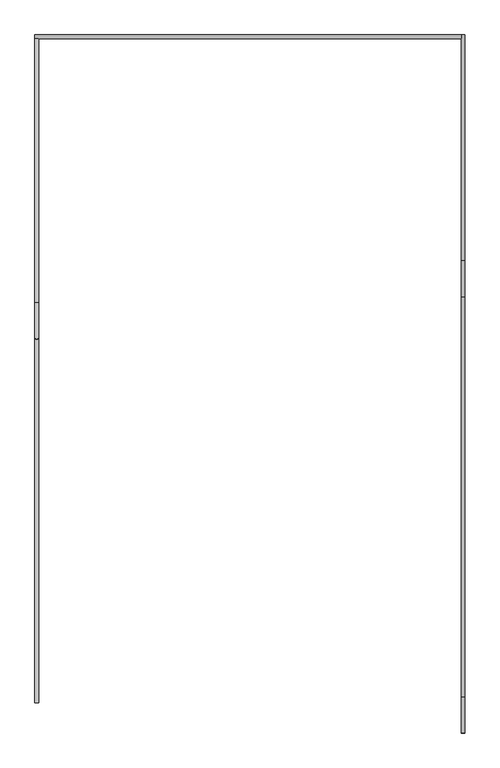
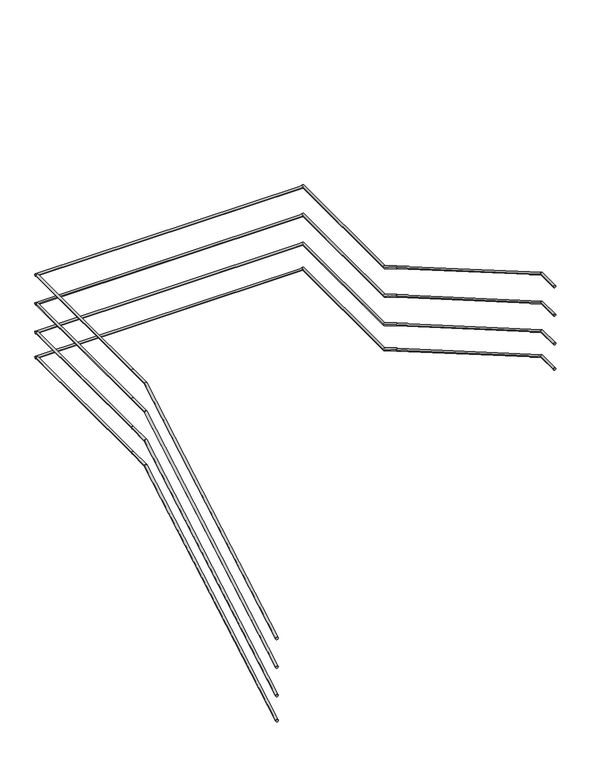
"""IFC4 building model written with IfcOpenShell, lengths in millimetres: railing geometry."""

import ifcopenshell
import ifcopenshell.guid

model = None  # the IFC model being written
_history = None  # IfcOwnerHistory: only IFC2X3 demands one
_inside = {}  # id of a spatial element -> (the spatial element, [elements in it])
_under = {}  # id of a project, library or spatial element -> (it, [spatial elements below it])
_declared = {}  # id of a project -> (the project, [libraries it declares])
_typed = {}  # id of a type object -> (the type object, [elements of that type])
_made_of = {}  # id of a material, layer set ... -> (it, [elements and type objects made of it])


def new_model(schema):
    """Start an empty IFC model of exactly this schema.

    Asked for "IFC4X3", IfcOpenShell would pick the latest addendum, in which some entities
    have other attributes; the version numbers below select the first issue.
    IFC2X3 requires an IfcOwnerHistory on every rooted entity: one is made here for all.
    """
    global model, _history
    if schema == "IFC4X3":
        model = ifcopenshell.file(schema_version=(4, 3, 0, 0))
    else:
        model = ifcopenshell.file(schema=schema)
    _inside.clear()
    _under.clear()
    _declared.clear()
    _typed.clear()
    _made_of.clear()
    _history = None
    if model.schema == "IFC2X3":
        org = make("IfcOrganization", Name="unknown")
        user = make(
            "IfcPersonAndOrganization",
            ThePerson=make("IfcPerson", FamilyName="unknown"),
            TheOrganization=org,
        )
        app = make(
            "IfcApplication",
            ApplicationDeveloper=org,
            Version="unknown",
            ApplicationFullName="unknown",
            ApplicationIdentifier="unknown",
        )
        _history = make(
            "IfcOwnerHistory",
            OwningUser=user,
            OwningApplication=app,
            ChangeAction="ADDED",
            CreationDate=0,
        )
    return model


def make(cls, **values):
    """One entity of the class cls with the attributes given. An attribute that is None is left unset."""
    return model.create_entity(
        cls, **{name: value for name, value in values.items() if value is not None}
    )


def rooted(cls, **values):
    """An entity with a GlobalId (a new one), such as an element, a storey or a relation."""
    return make(cls, GlobalId=ifcopenshell.guid.new(), OwnerHistory=_history, **values)


def si_unit(unit_type, name, prefix=None):
    """IfcSIUnit, for example si_unit("LENGTHUNIT", "METRE", prefix="MILLI")."""
    return make("IfcSIUnit", UnitType=unit_type, Prefix=prefix, Name=name)


def assignment(units):
    """IfcUnitAssignment: the units of a project."""
    return None if units is None else make("IfcUnitAssignment", Units=units)


def point(xyz):
    """IfcCartesianPoint."""
    return None if xyz is None else make("IfcCartesianPoint", Coordinates=xyz)


def direction(xyz):
    """IfcDirection."""
    return None if xyz is None else make("IfcDirection", DirectionRatios=xyz)


def frame(location, z_axis=None, x_axis=None):
    """IfcAxis2Placement3D, a coordinate frame: its origin and axes. An axis left out is left unset."""
    return make(
        "IfcAxis2Placement3D",
        Location=point(location),
        Axis=direction(z_axis),
        RefDirection=direction(x_axis),
    )


def origin():
    """The frame at (0, 0, 0) with its axes left unset."""
    return frame((0.0, 0.0, 0.0))


def place(relative_to, where):
    """IfcLocalPlacement: puts the frame where relative to a parent placement (None: the world)."""
    return make(
        "IfcLocalPlacement", PlacementRelTo=relative_to, RelativePlacement=where
    )


def context(
    kind, dimensions, precision=None, world=None, true_north=None, identifier=None
):
    """IfcGeometricRepresentationContext, for example the 3D "Model" context."""
    return make(
        "IfcGeometricRepresentationContext",
        ContextIdentifier=identifier,
        ContextType=kind,
        CoordinateSpaceDimension=dimensions,
        Precision=precision,
        WorldCoordinateSystem=world,
        TrueNorth=true_north,
    )


def project(units=None, contexts=None):
    """IfcProject with its units and contexts."""
    return rooted(
        "IfcProject",
        Name="project",
        RepresentationContexts=contexts,
        UnitsInContext=assignment(units),
    )


def spatial(cls, under=None, at=None, **own):
    """A site, building, storey or space (cls), placed at a placement, below another one or the project."""
    s = rooted(cls, ObjectPlacement=at, **own)
    if under is not None:
        _under.setdefault(under.id(), (under, []))[1].append(s)
    return s


def circle_curve(where, radius):
    """IfcCircle in the frame where."""
    return make("IfcCircle", Position=where, Radius=radius)


def ellipse_curve(where, semi_axis1, semi_axis2):
    """IfcEllipse in the frame where."""
    return make(
        "IfcEllipse", Position=where, SemiAxis1=semi_axis1, SemiAxis2=semi_axis2
    )


def shape(context_of_items, identifier, shape_type, items):
    """IfcShapeRepresentation: the items that make up one representation, for example the "Body"."""
    return make(
        "IfcShapeRepresentation",
        ContextOfItems=context_of_items,
        RepresentationIdentifier=identifier,
        RepresentationType=shape_type,
        Items=items,
    )


def source(mapping_origin, context_of_items, identifier, shape_type, items):
    """IfcRepresentationMap: a shape defined once, which mapped items show again and again."""
    return make(
        "IfcRepresentationMap",
        MappingOrigin=mapping_origin,
        MappedRepresentation=shape(context_of_items, identifier, shape_type, items),
    )


def transform(
    local_origin,
    x_axis=None,
    y_axis=None,
    z_axis=None,
    scale=None,
    scale2=None,
    scale3=None,
    uniform=True,
):
    """IfcCartesianTransformationOperator3D, or its non-uniform kind. x_axis, y_axis, z_axis: its Axis1, 2, 3."""
    if uniform:
        return make(
            "IfcCartesianTransformationOperator3D",
            Axis1=direction(x_axis),
            Axis2=direction(y_axis),
            LocalOrigin=point(local_origin),
            Scale=scale,
            Axis3=direction(z_axis),
        )
    return make(
        "IfcCartesianTransformationOperator3DnonUniform",
        Axis1=direction(x_axis),
        Axis2=direction(y_axis),
        LocalOrigin=point(local_origin),
        Scale=scale,
        Axis3=direction(z_axis),
        Scale2=scale2,
        Scale3=scale3,
    )


def mapped(mapping_source, mapping_target):
    """IfcMappedItem: shows the shape of a source again, moved by a transform."""
    return make(
        "IfcMappedItem", MappingSource=mapping_source, MappingTarget=mapping_target
    )


def made_of(thing, what):
    """Note that an element or type object is made of a material, layer set ...; save() writes the relation."""
    if what is not None:
        _made_of.setdefault(what.id(), (what, []))[1].append(thing)
    return thing


def element(
    cls,
    number,
    at=None,
    inside=None,
    cuts=None,
    type_object=None,
    material=None,
    context=None,
    identifier="Body",
    shape_type=None,
    held_by="IfcProductDefinitionShape",
    body=None,
    shapes=None,
    **own,
):
    """One element of the class cls, such as IfcWall. Its Tag is "e" and its number.

    at: its placement. inside: the storey or other place that contains it. cuts: it is an
    opening in that element (IfcRelVoidsElement). A single representation is given by context,
    identifier, shape_type and body (its items); several are given by shapes. held_by: the class
    of the entity that holds the representations. save() writes the other relations.
    """
    e = rooted(cls, Tag="e%d" % number, ObjectPlacement=at, **own)
    if body is not None:
        shapes = [shape(context, identifier, shape_type, body)]
    if shapes is not None:
        e.Representation = make(held_by, Representations=shapes)
    if inside is not None:
        _inside.setdefault(inside.id(), (inside, []))[1].append(e)
    if cuts is not None:
        rooted(
            "IfcRelVoidsElement", RelatingBuildingElement=cuts, RelatedOpeningElement=e
        )
    if type_object is not None:
        _typed.setdefault(type_object.id(), (type_object, []))[1].append(e)
    return made_of(e, material)


def aggregate(whole, parts):
    """IfcRelAggregates: a whole, such as a stair, and the parts it consists of."""
    return rooted("IfcRelAggregates", RelatingObject=whole, RelatedObjects=parts)


def save(model, path):
    """Write the relations noted so far, then the file.

    IfcRelAggregates (storeys below a building ...), IfcRelContainedInSpatialStructure (elements
    in a storey), IfcRelDefinesByType, IfcRelAssociatesMaterial and IfcRelDeclares: one each for
    every whole, place, type object, material and project.
    """
    for whole, parts in _under.values():
        aggregate(whole, parts)
    for where, things in _inside.values():
        rooted(
            "IfcRelContainedInSpatialStructure",
            RelatedElements=things,
            RelatingStructure=where,
        )
    for kind, things in _typed.values():
        rooted("IfcRelDefinesByType", RelatedObjects=things, RelatingType=kind)
    for what, things in _made_of.values():
        rooted("IfcRelAssociatesMaterial", RelatedObjects=things, RelatingMaterial=what)
    for by, libraries in _declared.values():
        rooted("IfcRelDeclares", RelatingContext=by, RelatedDefinitions=libraries)
    model.write(path)


def plane_surface(at):
    """IfcPlane: the flat surface through the origin of the frame at, square to its z axis."""
    return make("IfcPlane", Position=at)


def cylinder_surface(at, radius):
    """IfcCylindricalSurface: all points at the distance radius from the z axis of the frame at."""
    return make("IfcCylindricalSurface", Position=at, Radius=radius)


def advanced_brep(points, edges, surfaces, faces):
    """IfcAdvancedBrep: a solid bounded by faces that lie on surfaces and meet in shared edges.

    An edge is (start, end): straight between two places in points (the first is 0);
    or (start, end, curve); or (start, end, curve, False) where it runs against its curve.
    A face is (place in surfaces, loops), or (place, loops, False) where it looks against
    its surface's normal. A loop lists edges by number (the first is 1), with a minus sign
    where the edge is run from its end to its start. The first loop is the outer one.
    """
    corners = [point(p) for p in points]
    vertices = [make("IfcVertexPoint", VertexGeometry=c) for c in corners]
    made = []
    for start, end, *more in edges:
        made.append(
            make(
                "IfcEdgeCurve",
                EdgeStart=vertices[start],
                EdgeEnd=vertices[end],
                EdgeGeometry=more[0] if more else make("IfcPolyline", Points=[corners[start], corners[end]]),
                SameSense=more[1] if len(more) > 1 else True,
            )
        )
    hull = []
    for where, loops, *sense in faces:
        bounds = []
        for j, loop in enumerate(loops):
            ring = [make("IfcOrientedEdge", EdgeElement=made[abs(k) - 1], Orientation=k > 0) for k in loop]
            bounds.append(
                make(
                    "IfcFaceOuterBound" if j == 0 else "IfcFaceBound",
                    Bound=make("IfcEdgeLoop", EdgeList=ring),
                    Orientation=True,
                )
            )
        hull.append(make("IfcAdvancedFace", Bounds=bounds, FaceSurface=surfaces[where], SameSense=sense[0] if sense else True))
    return make("IfcAdvancedBrep", Outer=make("IfcClosedShell", CfsFaces=hull))


def railing_27d6a30b(model_context):
    return source(origin(), model_context, "Body", "AdvancedBrep", [
        advanced_brep(
        [(51115.4, 12029.5208589, 12766.5366726), (51085.4, 12029.5208589, 12766.5366726), (51115.4, 15033.554313, 14508.0053416), (51085.4, 15033.554313, 14508.0053416), (51115.4, 15329.5208589, 14508.0053416), (51085.4, 15329.5208589, 14508.0053416)],
        [
            (0, 1, ellipse_curve(frame((51100.4, 12029.5208589, 12766.5366726), z_axis=(0.0, -1.0, 0.0), x_axis=(0.0, 0.0, -1.0)), 17.3382342, 15.0)),
            (1, 0, ellipse_curve(frame((51100.4, 12029.5208589, 12766.5366726), z_axis=(0.0, -1.0, 0.0), x_axis=(0.0, 0.0, -1.0)), 17.3382342, 15.0)),
            (0, 2),
            (2, 3, ellipse_curve(frame((51100.4, 15033.554313, 14508.0053416), z_axis=(0.0, -0.9656966401166088, -0.25967286971782944), x_axis=(0.0, 0.25967286971782905, -0.9656966401166089)), 15.5328282, 15.0)),
            (3, 1),
            (3, 2, ellipse_curve(frame((51100.4, 15033.554313, 14508.0053416), z_axis=(0.0, -0.9656966401166088, -0.25967286971782944), x_axis=(0.0, 0.25967286971782905, -0.9656966401166089)), 15.5328282, 15.0)),
            (4, 5, circle_curve(frame((51100.4, 15329.5208589, 14508.0053416), z_axis=(0.0, 1.0, 0.0), x_axis=(-1.0, 0.0, 0.0)), 15.0)),
            (5, 4, circle_curve(frame((51100.4, 15329.5208589, 14508.0053416), z_axis=(0.0, 1.0, 0.0), x_axis=(-1.0, 0.0, 0.0)), 15.0)),
            (2, 4),
            (5, 3),
        ],
        [
            plane_surface(frame((51100.4, 12029.5208589, 12783.8749068), z_axis=(0.0, -1.0, 0.0), x_axis=(0.0, 0.0, 1.0))),
            cylinder_surface(frame((51100.4, 12037.0438154, 12770.8978068), z_axis=(0.0, -0.8651400014650144, -0.5015304356318916), x_axis=(-1.0, 0.0, 0.0)), 15.0),
            plane_surface(frame((51100.4, 15329.5208589, 14523.0053416), z_axis=(0.0, 1.0, 0.0), x_axis=(0.0, 0.0, 1.0))),
            cylinder_surface(frame((51100.4, 15029.5208589, 14508.0053416), z_axis=(0.0, -1.0, 0.0), x_axis=(-1.0, 0.0, 0.0)), 15.0),
        ],
        [
            (0, [[1, 2]]),
            (1, [[-1, 3, 4, 5]]),
            (1, [[-2, -5, 6, -3]]),
            (2, [[7, 8]]),
            (3, [[-4, 9, -8, 10]]),
            (3, [[-6, -10, -7, -9]]),
        ],
    ),
        advanced_brep(
        [(51115.4, 15329.5208589, 14508.0053416), (51085.4, 15329.5208589, 14508.0053416), (51115.4, 17509.1208589, 14508.0053416), (51085.4, 17509.1208589, 14508.0053416)],
        [
            (0, 1, circle_curve(frame((51100.4, 15329.5208589, 14508.0053416), z_axis=(0.0, -1.0, 0.0), x_axis=(-1.0, 0.0, 0.0)), 15.0)),
            (1, 0, circle_curve(frame((51100.4, 15329.5208589, 14508.0053416), z_axis=(0.0, -1.0, 0.0), x_axis=(-1.0, 0.0, 0.0)), 15.0)),
            (2, 3, circle_curve(frame((51100.4, 17509.1208589, 14508.0053416), z_axis=(0.0, 1.0, 0.0), x_axis=(-1.0, 0.0, 0.0)), 15.0)),
            (3, 2, circle_curve(frame((51100.4, 17509.1208589, 14508.0053416), z_axis=(0.0, 1.0, 0.0), x_axis=(-1.0, 0.0, 0.0)), 15.0)),
            (0, 2),
            (3, 1),
        ],
        [
            plane_surface(frame((51100.4, 15329.5208589, 14523.0053416), z_axis=(0.0, -1.0, 0.0), x_axis=(0.0, 0.0, 1.0))),
            plane_surface(frame((51100.4, 17509.1208589, 14523.0053416), z_axis=(0.0, 1.0, 0.0), x_axis=(0.0, 0.0, 1.0))),
            cylinder_surface(frame((51100.4, 15329.5208589, 14508.0053416), z_axis=(0.0, -1.0, 0.0), x_axis=(-1.0, 0.0, 0.0)), 15.0),
        ],
        [
            (0, [[1, 2]]),
            (1, [[3, 4]]),
            (2, [[-1, 5, -4, 6]]),
            (2, [[-2, -6, -3, -5]]),
        ],
    ),
        advanced_brep(
        [(51085.4, 17509.1208589, 14508.0053416), (51085.4, 17539.1208589, 14508.0053416), (54606.835546, 17509.1208589, 14508.0053416), (54606.835546, 17539.1208589, 14508.0053416)],
        [
            (0, 1, circle_curve(frame((51085.4, 17524.1208589, 14508.0053416), z_axis=(-1.0, 0.0, 0.0), x_axis=(0.0, 1.0, 0.0)), 15.0)),
            (1, 0, circle_curve(frame((51085.4, 17524.1208589, 14508.0053416), z_axis=(-1.0, 0.0, 0.0), x_axis=(0.0, 1.0, 0.0)), 15.0)),
            (2, 3, circle_curve(frame((54606.835546, 17524.1208589, 14508.0053416), z_axis=(1.0, 0.0, 0.0), x_axis=(0.0, 1.0, 0.0)), 15.0)),
            (3, 2, circle_curve(frame((54606.835546, 17524.1208589, 14508.0053416), z_axis=(1.0, 0.0, 0.0), x_axis=(0.0, 1.0, 0.0)), 15.0)),
            (0, 2),
            (3, 1),
        ],
        [
            plane_surface(frame((51085.4, 17524.1208589, 14523.0053416), z_axis=(-1.0, 0.0, 0.0), x_axis=(0.0, 1.0, 0.0))),
            plane_surface(frame((54606.835546, 17524.1208589, 14523.0053416), z_axis=(1.0, 0.0, 0.0), x_axis=(0.0, 1.0, 0.0))),
            cylinder_surface(frame((51085.4, 17524.1208589, 14508.0053416), z_axis=(-1.0, 0.0, 0.0), x_axis=(0.0, 1.0, 0.0)), 15.0),
        ],
        [
            (0, [[1, 2]]),
            (1, [[3, 4]]),
            (2, [[-1, 5, -4, 6]]),
            (2, [[-2, -6, -3, -5]]),
        ],
    ),
        advanced_brep(
        [(54606.835546, 17539.1208589, 14508.0053416), (54636.835546, 17539.1208589, 14508.0053416), (54606.835546, 15675.4874048, 14508.0053416), (54636.835546, 15675.4874048, 14508.0053416), (54606.835546, 15379.5208589, 14679.5801509), (54636.835546, 15379.5208589, 14679.5801509)],
        [
            (0, 1, circle_curve(frame((54621.835546, 17539.1208589, 14508.0053416), z_axis=(0.0, 1.0, 0.0), x_axis=(1.0, 0.0, 0.0)), 15.0)),
            (1, 0, circle_curve(frame((54621.835546, 17539.1208589, 14508.0053416), z_axis=(0.0, 1.0, 0.0), x_axis=(1.0, 0.0, 0.0)), 15.0)),
            (0, 2),
            (2, 3, ellipse_curve(frame((54621.835546, 15675.4874048, 14508.0053416), z_axis=(0.0, 0.9656966401166088, -0.25967286971782944), x_axis=(0.0, 0.2596728697178298, 0.9656966401166087)), 15.5328282, 15.0)),
            (3, 1),
            (3, 2, ellipse_curve(frame((54621.835546, 15675.4874048, 14508.0053416), z_axis=(0.0, 0.9656966401166088, -0.25967286971782944), x_axis=(0.0, 0.2596728697178298, 0.9656966401166087)), 15.5328282, 15.0)),
            (4, 5, ellipse_curve(frame((54621.835546, 15379.5208589, 14679.5801509), z_axis=(0.0, -1.0, 0.0), x_axis=(0.0, 0.0, -1.0)), 17.3382342, 15.0)),
            (5, 4, ellipse_curve(frame((54621.835546, 15379.5208589, 14679.5801509), z_axis=(0.0, -1.0, 0.0), x_axis=(0.0, 0.0, -1.0)), 17.3382342, 15.0)),
            (2, 4),
            (5, 3),
        ],
        [
            plane_surface(frame((54621.835546, 17539.1208589, 14523.0053416), z_axis=(0.0, 1.0, 0.0), x_axis=(0.0, 0.0, -1.0))),
            cylinder_surface(frame((54621.835546, 17539.1208589, 14508.0053416), z_axis=(0.0, 1.0, 0.0), x_axis=(1.0, 0.0, 0.0)), 15.0),
            plane_surface(frame((54621.835546, 15379.5208589, 14696.9183851), z_axis=(0.0, -1.0, 0.0), x_axis=(0.0, 0.0, -1.0))),
            cylinder_surface(frame((54621.835546, 15671.9979024, 14510.0282416), z_axis=(0.0, 0.8651400014650144, -0.5015304356318916), x_axis=(1.0, 0.0, 0.0)), 15.0),
        ],
        [
            (0, [[1, 2]]),
            (1, [[-1, 3, 4, 5]]),
            (1, [[-2, -5, 6, -3]]),
            (2, [[7, 8]]),
            (3, [[-4, 9, -8, 10]]),
            (3, [[-6, -10, -7, -9]]),
        ],
    ),
        advanced_brep(
        [(54606.835546, 15379.5208589, 14679.5801509), (54636.835546, 15379.5208589, 14679.5801509), (54606.835546, 12075.4874048, 16594.9618634), (54636.835546, 12075.4874048, 16594.9618634), (54606.835546, 11779.5208589, 16594.9618634), (54636.835546, 11779.5208589, 16594.9618634)],
        [
            (0, 1, ellipse_curve(frame((54621.835546, 15379.5208589, 14679.5801509), z_axis=(0.0, 1.0, 0.0), x_axis=(0.0, 0.0, -1.0)), 17.3382342, 15.0)),
            (1, 0, ellipse_curve(frame((54621.835546, 15379.5208589, 14679.5801509), z_axis=(0.0, 1.0, 0.0), x_axis=(0.0, 0.0, -1.0)), 17.3382342, 15.0)),
            (0, 2),
            (2, 3, ellipse_curve(frame((54621.835546, 12075.4874048, 16594.9618634), z_axis=(0.0, 0.9656966401166087, -0.2596728697178297), x_axis=(0.0, -0.259672869717829, -0.9656966401166089)), 15.5328282, 15.0)),
            (3, 1),
            (3, 2, ellipse_curve(frame((54621.835546, 12075.4874048, 16594.9618634), z_axis=(0.0, 0.9656966401166087, -0.2596728697178297), x_axis=(0.0, -0.259672869717829, -0.9656966401166089)), 15.5328282, 15.0)),
            (4, 5, circle_curve(frame((54621.835546, 11779.5208589, 16594.9618634), z_axis=(0.0, -1.0, 0.0), x_axis=(1.0, 0.0, 0.0)), 15.0)),
            (5, 4, circle_curve(frame((54621.835546, 11779.5208589, 16594.9618634), z_axis=(0.0, -1.0, 0.0), x_axis=(1.0, 0.0, 0.0)), 15.0)),
            (2, 4),
            (5, 3),
        ],
        [
            plane_surface(frame((54621.835546, 15379.5208589, 14696.9183851), z_axis=(0.0, 1.0, 0.0), x_axis=(0.0, 0.0, -1.0))),
            cylinder_surface(frame((54621.835546, 15371.9979024, 14683.9412851), z_axis=(0.0, 0.865140001465014, -0.5015304356318923), x_axis=(1.0, 0.0, 0.0)), 15.0),
            plane_surface(frame((54621.835546, 11779.5208589, 16609.9618634), z_axis=(0.0, -1.0, 0.0), x_axis=(0.0, 0.0, -1.0))),
            cylinder_surface(frame((54621.835546, 12079.5208589, 16594.9618634), z_axis=(0.0, 1.0, 0.0), x_axis=(1.0, 0.0, 0.0)), 15.0),
        ],
        [
            (0, [[1, 2]]),
            (1, [[-1, 3, 4, 5]]),
            (1, [[-2, -5, 6, -3]]),
            (2, [[7, 8]]),
            (3, [[-4, 9, -8, 10]]),
            (3, [[-6, -10, -7, -9]]),
        ],
    ),
        advanced_brep(
        [(51115.4, 12029.5208589, 11966.5366726), (51085.4, 12029.5208589, 11966.5366726), (51115.4, 15033.554313, 13708.0053416), (51085.4, 15033.554313, 13708.0053416), (51115.4, 15329.5208589, 13708.0053416), (51085.4, 15329.5208589, 13708.0053416)],
        [
            (0, 1, ellipse_curve(frame((51100.4, 12029.5208589, 11966.5366726), z_axis=(0.0, -1.0, 0.0), x_axis=(0.0, 0.0, -1.0)), 17.3382342, 15.0)),
            (1, 0, ellipse_curve(frame((51100.4, 12029.5208589, 11966.5366726), z_axis=(0.0, -1.0, 0.0), x_axis=(0.0, 0.0, -1.0)), 17.3382342, 15.0)),
            (0, 2),
            (2, 3, ellipse_curve(frame((51100.4, 15033.554313, 13708.0053416), z_axis=(0.0, -0.9656966401166088, -0.25967286971782944), x_axis=(0.0, 0.25967286971782905, -0.9656966401166089)), 15.5328282, 15.0)),
            (3, 1),
            (3, 2, ellipse_curve(frame((51100.4, 15033.554313, 13708.0053416), z_axis=(0.0, -0.9656966401166088, -0.25967286971782944), x_axis=(0.0, 0.25967286971782905, -0.9656966401166089)), 15.5328282, 15.0)),
            (4, 5, circle_curve(frame((51100.4, 15329.5208589, 13708.0053416), z_axis=(0.0, 1.0, 0.0), x_axis=(-1.0, 0.0, 0.0)), 15.0)),
            (5, 4, circle_curve(frame((51100.4, 15329.5208589, 13708.0053416), z_axis=(0.0, 1.0, 0.0), x_axis=(-1.0, 0.0, 0.0)), 15.0)),
            (2, 4),
            (5, 3),
        ],
        [
            plane_surface(frame((51100.4, 12029.5208589, 11983.8749068), z_axis=(0.0, -1.0, 0.0), x_axis=(0.0, 0.0, 1.0))),
            cylinder_surface(frame((51100.4, 12037.0438154, 11970.8978068), z_axis=(0.0, -0.8651400014650144, -0.5015304356318916), x_axis=(-1.0, 0.0, 0.0)), 15.0),
            plane_surface(frame((51100.4, 15329.5208589, 13723.0053416), z_axis=(0.0, 1.0, 0.0), x_axis=(0.0, 0.0, 1.0))),
            cylinder_surface(frame((51100.4, 15029.5208589, 13708.0053416), z_axis=(0.0, -1.0, 0.0), x_axis=(-1.0, 0.0, 0.0)), 15.0),
        ],
        [
            (0, [[1, 2]]),
            (1, [[-1, 3, 4, 5]]),
            (1, [[-2, -5, 6, -3]]),
            (2, [[7, 8]]),
            (3, [[-4, 9, -8, 10]]),
            (3, [[-6, -10, -7, -9]]),
        ],
    ),
        advanced_brep(
        [(51115.4, 15329.5208589, 13708.0053416), (51085.4, 15329.5208589, 13708.0053416), (51115.4, 17509.1208589, 13708.0053416), (51085.4, 17509.1208589, 13708.0053416)],
        [
            (0, 1, circle_curve(frame((51100.4, 15329.5208589, 13708.0053416), z_axis=(0.0, -1.0, 0.0), x_axis=(-1.0, 0.0, 0.0)), 15.0)),
            (1, 0, circle_curve(frame((51100.4, 15329.5208589, 13708.0053416), z_axis=(0.0, -1.0, 0.0), x_axis=(-1.0, 0.0, 0.0)), 15.0)),
            (2, 3, circle_curve(frame((51100.4, 17509.1208589, 13708.0053416), z_axis=(0.0, 1.0, 0.0), x_axis=(-1.0, 0.0, 0.0)), 15.0)),
            (3, 2, circle_curve(frame((51100.4, 17509.1208589, 13708.0053416), z_axis=(0.0, 1.0, 0.0), x_axis=(-1.0, 0.0, 0.0)), 15.0)),
            (0, 2),
            (3, 1),
        ],
        [
            plane_surface(frame((51100.4, 15329.5208589, 13723.0053416), z_axis=(0.0, -1.0, 0.0), x_axis=(0.0, 0.0, 1.0))),
            plane_surface(frame((51100.4, 17509.1208589, 13723.0053416), z_axis=(0.0, 1.0, 0.0), x_axis=(0.0, 0.0, 1.0))),
            cylinder_surface(frame((51100.4, 15329.5208589, 13708.0053416), z_axis=(0.0, -1.0, 0.0), x_axis=(-1.0, 0.0, 0.0)), 15.0),
        ],
        [
            (0, [[1, 2]]),
            (1, [[3, 4]]),
            (2, [[-1, 5, -4, 6]]),
            (2, [[-2, -6, -3, -5]]),
        ],
    ),
        advanced_brep(
        [(51085.4, 17509.1208589, 13708.0053416), (51085.4, 17539.1208589, 13708.0053416), (54606.835546, 17509.1208589, 13708.0053416), (54606.835546, 17539.1208589, 13708.0053416)],
        [
            (0, 1, circle_curve(frame((51085.4, 17524.1208589, 13708.0053416), z_axis=(-1.0, 0.0, 0.0), x_axis=(0.0, 1.0, 0.0)), 15.0)),
            (1, 0, circle_curve(frame((51085.4, 17524.1208589, 13708.0053416), z_axis=(-1.0, 0.0, 0.0), x_axis=(0.0, 1.0, 0.0)), 15.0)),
            (2, 3, circle_curve(frame((54606.835546, 17524.1208589, 13708.0053416), z_axis=(1.0, 0.0, 0.0), x_axis=(0.0, 1.0, 0.0)), 15.0)),
            (3, 2, circle_curve(frame((54606.835546, 17524.1208589, 13708.0053416), z_axis=(1.0, 0.0, 0.0), x_axis=(0.0, 1.0, 0.0)), 15.0)),
            (0, 2),
            (3, 1),
        ],
        [
            plane_surface(frame((51085.4, 17524.1208589, 13723.0053416), z_axis=(-1.0, 0.0, 0.0), x_axis=(0.0, 1.0, 0.0))),
            plane_surface(frame((54606.835546, 17524.1208589, 13723.0053416), z_axis=(1.0, 0.0, 0.0), x_axis=(0.0, 1.0, 0.0))),
            cylinder_surface(frame((51085.4, 17524.1208589, 13708.0053416), z_axis=(-1.0, 0.0, 0.0), x_axis=(0.0, 1.0, 0.0)), 15.0),
        ],
        [
            (0, [[1, 2]]),
            (1, [[3, 4]]),
            (2, [[-1, 5, -4, 6]]),
            (2, [[-2, -6, -3, -5]]),
        ],
    ),
        advanced_brep(
        [(54606.835546, 17539.1208589, 13708.0053416), (54636.835546, 17539.1208589, 13708.0053416), (54606.835546, 15675.4874048, 13708.0053416), (54636.835546, 15675.4874048, 13708.0053416), (54606.835546, 15379.5208589, 13879.5801509), (54636.835546, 15379.5208589, 13879.5801509)],
        [
            (0, 1, circle_curve(frame((54621.835546, 17539.1208589, 13708.0053416), z_axis=(0.0, 1.0, 0.0), x_axis=(1.0, 0.0, 0.0)), 15.0)),
            (1, 0, circle_curve(frame((54621.835546, 17539.1208589, 13708.0053416), z_axis=(0.0, 1.0, 0.0), x_axis=(1.0, 0.0, 0.0)), 15.0)),
            (0, 2),
            (2, 3, ellipse_curve(frame((54621.835546, 15675.4874048, 13708.0053416), z_axis=(0.0, 0.9656966401166088, -0.25967286971782944), x_axis=(0.0, 0.2596728697178298, 0.9656966401166087)), 15.5328282, 15.0)),
            (3, 1),
            (3, 2, ellipse_curve(frame((54621.835546, 15675.4874048, 13708.0053416), z_axis=(0.0, 0.9656966401166088, -0.25967286971782944), x_axis=(0.0, 0.2596728697178298, 0.9656966401166087)), 15.5328282, 15.0)),
            (4, 5, ellipse_curve(frame((54621.835546, 15379.5208589, 13879.5801509), z_axis=(0.0, -1.0, 0.0), x_axis=(0.0, 0.0, -1.0)), 17.3382342, 15.0)),
            (5, 4, ellipse_curve(frame((54621.835546, 15379.5208589, 13879.5801509), z_axis=(0.0, -1.0, 0.0), x_axis=(0.0, 0.0, -1.0)), 17.3382342, 15.0)),
            (2, 4),
            (5, 3),
        ],
        [
            plane_surface(frame((54621.835546, 17539.1208589, 13723.0053416), z_axis=(0.0, 1.0, 0.0), x_axis=(0.0, 0.0, -1.0))),
            cylinder_surface(frame((54621.835546, 17539.1208589, 13708.0053416), z_axis=(0.0, 1.0, 0.0), x_axis=(1.0, 0.0, 0.0)), 15.0),
            plane_surface(frame((54621.835546, 15379.5208589, 13896.9183851), z_axis=(0.0, -1.0, 0.0), x_axis=(0.0, 0.0, -1.0))),
            cylinder_surface(frame((54621.835546, 15671.9979024, 13710.0282416), z_axis=(0.0, 0.8651400014650144, -0.5015304356318916), x_axis=(1.0, 0.0, 0.0)), 15.0),
        ],
        [
            (0, [[1, 2]]),
            (1, [[-1, 3, 4, 5]]),
            (1, [[-2, -5, 6, -3]]),
            (2, [[7, 8]]),
            (3, [[-4, 9, -8, 10]]),
            (3, [[-6, -10, -7, -9]]),
        ],
    ),
        advanced_brep(
        [(54606.835546, 15379.5208589, 13879.5801509), (54636.835546, 15379.5208589, 13879.5801509), (54606.835546, 12075.4874048, 15794.9618634), (54636.835546, 12075.4874048, 15794.9618634), (54606.835546, 11779.5208589, 15794.9618634), (54636.835546, 11779.5208589, 15794.9618634)],
        [
            (0, 1, ellipse_curve(frame((54621.835546, 15379.5208589, 13879.5801509), z_axis=(0.0, 1.0, 0.0), x_axis=(0.0, 0.0, -1.0)), 17.3382342, 15.0)),
            (1, 0, ellipse_curve(frame((54621.835546, 15379.5208589, 13879.5801509), z_axis=(0.0, 1.0, 0.0), x_axis=(0.0, 0.0, -1.0)), 17.3382342, 15.0)),
            (0, 2),
            (2, 3, ellipse_curve(frame((54621.835546, 12075.4874048, 15794.9618634), z_axis=(0.0, 0.9656966401166087, -0.2596728697178297), x_axis=(0.0, -0.259672869717829, -0.9656966401166089)), 15.5328282, 15.0)),
            (3, 1),
            (3, 2, ellipse_curve(frame((54621.835546, 12075.4874048, 15794.9618634), z_axis=(0.0, 0.9656966401166087, -0.2596728697178297), x_axis=(0.0, -0.259672869717829, -0.9656966401166089)), 15.5328282, 15.0)),
            (4, 5, circle_curve(frame((54621.835546, 11779.5208589, 15794.9618634), z_axis=(0.0, -1.0, 0.0), x_axis=(1.0, 0.0, 0.0)), 15.0)),
            (5, 4, circle_curve(frame((54621.835546, 11779.5208589, 15794.9618634), z_axis=(0.0, -1.0, 0.0), x_axis=(1.0, 0.0, 0.0)), 15.0)),
            (2, 4),
            (5, 3),
        ],
        [
            plane_surface(frame((54621.835546, 15379.5208589, 13896.9183851), z_axis=(0.0, 1.0, 0.0), x_axis=(0.0, 0.0, -1.0))),
            cylinder_surface(frame((54621.835546, 15371.9979024, 13883.9412851), z_axis=(0.0, 0.865140001465014, -0.5015304356318923), x_axis=(1.0, 0.0, 0.0)), 15.0),
            plane_surface(frame((54621.835546, 11779.5208589, 15809.9618634), z_axis=(0.0, -1.0, 0.0), x_axis=(0.0, 0.0, -1.0))),
            cylinder_surface(frame((54621.835546, 12079.5208589, 15794.9618634), z_axis=(0.0, 1.0, 0.0), x_axis=(1.0, 0.0, 0.0)), 15.0),
        ],
        [
            (0, [[1, 2]]),
            (1, [[-1, 3, 4, 5]]),
            (1, [[-2, -5, 6, -3]]),
            (2, [[7, 8]]),
            (3, [[-4, 9, -8, 10]]),
            (3, [[-6, -10, -7, -9]]),
        ],
    ),
        advanced_brep(
        [(51115.4, 12029.5208589, 12366.5366726), (51085.4, 12029.5208589, 12366.5366726), (51115.4, 15033.554313, 14108.0053416), (51085.4, 15033.554313, 14108.0053416), (51115.4, 15329.5208589, 14108.0053416), (51085.4, 15329.5208589, 14108.0053416)],
        [
            (0, 1, ellipse_curve(frame((51100.4, 12029.5208589, 12366.5366726), z_axis=(0.0, -1.0, 0.0), x_axis=(0.0, 0.0, -1.0)), 17.3382342, 15.0)),
            (1, 0, ellipse_curve(frame((51100.4, 12029.5208589, 12366.5366726), z_axis=(0.0, -1.0, 0.0), x_axis=(0.0, 0.0, -1.0)), 17.3382342, 15.0)),
            (0, 2),
            (2, 3, ellipse_curve(frame((51100.4, 15033.554313, 14108.0053416), z_axis=(0.0, -0.9656966401166088, -0.25967286971782944), x_axis=(0.0, 0.25967286971782905, -0.9656966401166089)), 15.5328282, 15.0)),
            (3, 1),
            (3, 2, ellipse_curve(frame((51100.4, 15033.554313, 14108.0053416), z_axis=(0.0, -0.9656966401166088, -0.25967286971782944), x_axis=(0.0, 0.25967286971782905, -0.9656966401166089)), 15.5328282, 15.0)),
            (4, 5, circle_curve(frame((51100.4, 15329.5208589, 14108.0053416), z_axis=(0.0, 1.0, 0.0), x_axis=(-1.0, 0.0, 0.0)), 15.0)),
            (5, 4, circle_curve(frame((51100.4, 15329.5208589, 14108.0053416), z_axis=(0.0, 1.0, 0.0), x_axis=(-1.0, 0.0, 0.0)), 15.0)),
            (2, 4),
            (5, 3),
        ],
        [
            plane_surface(frame((51100.4, 12029.5208589, 12383.8749068), z_axis=(0.0, -1.0, 0.0), x_axis=(0.0, 0.0, 1.0))),
            cylinder_surface(frame((51100.4, 12037.0438154, 12370.8978068), z_axis=(0.0, -0.8651400014650144, -0.5015304356318916), x_axis=(-1.0, 0.0, 0.0)), 15.0),
            plane_surface(frame((51100.4, 15329.5208589, 14123.0053416), z_axis=(0.0, 1.0, 0.0), x_axis=(0.0, 0.0, 1.0))),
            cylinder_surface(frame((51100.4, 15029.5208589, 14108.0053416), z_axis=(0.0, -1.0, 0.0), x_axis=(-1.0, 0.0, 0.0)), 15.0),
        ],
        [
            (0, [[1, 2]]),
            (1, [[-1, 3, 4, 5]]),
            (1, [[-2, -5, 6, -3]]),
            (2, [[7, 8]]),
            (3, [[-4, 9, -8, 10]]),
            (3, [[-6, -10, -7, -9]]),
        ],
    ),
        advanced_brep(
        [(51115.4, 15329.5208589, 14108.0053416), (51085.4, 15329.5208589, 14108.0053416), (51115.4, 17509.1208589, 14108.0053416), (51085.4, 17509.1208589, 14108.0053416)],
        [
            (0, 1, circle_curve(frame((51100.4, 15329.5208589, 14108.0053416), z_axis=(0.0, -1.0, 0.0), x_axis=(-1.0, 0.0, 0.0)), 15.0)),
            (1, 0, circle_curve(frame((51100.4, 15329.5208589, 14108.0053416), z_axis=(0.0, -1.0, 0.0), x_axis=(-1.0, 0.0, 0.0)), 15.0)),
            (2, 3, circle_curve(frame((51100.4, 17509.1208589, 14108.0053416), z_axis=(0.0, 1.0, 0.0), x_axis=(-1.0, 0.0, 0.0)), 15.0)),
            (3, 2, circle_curve(frame((51100.4, 17509.1208589, 14108.0053416), z_axis=(0.0, 1.0, 0.0), x_axis=(-1.0, 0.0, 0.0)), 15.0)),
            (0, 2),
            (3, 1),
        ],
        [
            plane_surface(frame((51100.4, 15329.5208589, 14123.0053416), z_axis=(0.0, -1.0, 0.0), x_axis=(0.0, 0.0, 1.0))),
            plane_surface(frame((51100.4, 17509.1208589, 14123.0053416), z_axis=(0.0, 1.0, 0.0), x_axis=(0.0, 0.0, 1.0))),
            cylinder_surface(frame((51100.4, 15329.5208589, 14108.0053416), z_axis=(0.0, -1.0, 0.0), x_axis=(-1.0, 0.0, 0.0)), 15.0),
        ],
        [
            (0, [[1, 2]]),
            (1, [[3, 4]]),
            (2, [[-1, 5, -4, 6]]),
            (2, [[-2, -6, -3, -5]]),
        ],
    ),
        advanced_brep(
        [(51085.4, 17509.1208589, 14108.0053416), (51085.4, 17539.1208589, 14108.0053416), (54606.835546, 17509.1208589, 14108.0053416), (54606.835546, 17539.1208589, 14108.0053416)],
        [
            (0, 1, circle_curve(frame((51085.4, 17524.1208589, 14108.0053416), z_axis=(-1.0, 0.0, 0.0), x_axis=(0.0, 1.0, 0.0)), 15.0)),
            (1, 0, circle_curve(frame((51085.4, 17524.1208589, 14108.0053416), z_axis=(-1.0, 0.0, 0.0), x_axis=(0.0, 1.0, 0.0)), 15.0)),
            (2, 3, circle_curve(frame((54606.835546, 17524.1208589, 14108.0053416), z_axis=(1.0, 0.0, 0.0), x_axis=(0.0, 1.0, 0.0)), 15.0)),
            (3, 2, circle_curve(frame((54606.835546, 17524.1208589, 14108.0053416), z_axis=(1.0, 0.0, 0.0), x_axis=(0.0, 1.0, 0.0)), 15.0)),
            (0, 2),
            (3, 1),
        ],
        [
            plane_surface(frame((51085.4, 17524.1208589, 14123.0053416), z_axis=(-1.0, 0.0, 0.0), x_axis=(0.0, 1.0, 0.0))),
            plane_surface(frame((54606.835546, 17524.1208589, 14123.0053416), z_axis=(1.0, 0.0, 0.0), x_axis=(0.0, 1.0, 0.0))),
            cylinder_surface(frame((51085.4, 17524.1208589, 14108.0053416), z_axis=(-1.0, 0.0, 0.0), x_axis=(0.0, 1.0, 0.0)), 15.0),
        ],
        [
            (0, [[1, 2]]),
            (1, [[3, 4]]),
            (2, [[-1, 5, -4, 6]]),
            (2, [[-2, -6, -3, -5]]),
        ],
    ),
        advanced_brep(
        [(54606.835546, 17539.1208589, 14108.0053416), (54636.835546, 17539.1208589, 14108.0053416), (54606.835546, 15675.4874048, 14108.0053416), (54636.835546, 15675.4874048, 14108.0053416), (54606.835546, 15379.5208589, 14279.5801509), (54636.835546, 15379.5208589, 14279.5801509)],
        [
            (0, 1, circle_curve(frame((54621.835546, 17539.1208589, 14108.0053416), z_axis=(0.0, 1.0, 0.0), x_axis=(1.0, 0.0, 0.0)), 15.0)),
            (1, 0, circle_curve(frame((54621.835546, 17539.1208589, 14108.0053416), z_axis=(0.0, 1.0, 0.0), x_axis=(1.0, 0.0, 0.0)), 15.0)),
            (0, 2),
            (2, 3, ellipse_curve(frame((54621.835546, 15675.4874048, 14108.0053416), z_axis=(0.0, 0.9656966401166088, -0.25967286971782944), x_axis=(0.0, 0.2596728697178298, 0.9656966401166087)), 15.5328282, 15.0)),
            (3, 1),
            (3, 2, ellipse_curve(frame((54621.835546, 15675.4874048, 14108.0053416), z_axis=(0.0, 0.9656966401166088, -0.25967286971782944), x_axis=(0.0, 0.2596728697178298, 0.9656966401166087)), 15.5328282, 15.0)),
            (4, 5, ellipse_curve(frame((54621.835546, 15379.5208589, 14279.5801509), z_axis=(0.0, -1.0, 0.0), x_axis=(0.0, 0.0, -1.0)), 17.3382342, 15.0)),
            (5, 4, ellipse_curve(frame((54621.835546, 15379.5208589, 14279.5801509), z_axis=(0.0, -1.0, 0.0), x_axis=(0.0, 0.0, -1.0)), 17.3382342, 15.0)),
            (2, 4),
            (5, 3),
        ],
        [
            plane_surface(frame((54621.835546, 17539.1208589, 14123.0053416), z_axis=(0.0, 1.0, 0.0), x_axis=(0.0, 0.0, -1.0))),
            cylinder_surface(frame((54621.835546, 17539.1208589, 14108.0053416), z_axis=(0.0, 1.0, 0.0), x_axis=(1.0, 0.0, 0.0)), 15.0),
            plane_surface(frame((54621.835546, 15379.5208589, 14296.9183851), z_axis=(0.0, -1.0, 0.0), x_axis=(0.0, 0.0, -1.0))),
            cylinder_surface(frame((54621.835546, 15671.9979024, 14110.0282416), z_axis=(0.0, 0.8651400014650144, -0.5015304356318916), x_axis=(1.0, 0.0, 0.0)), 15.0),
        ],
        [
            (0, [[1, 2]]),
            (1, [[-1, 3, 4, 5]]),
            (1, [[-2, -5, 6, -3]]),
            (2, [[7, 8]]),
            (3, [[-4, 9, -8, 10]]),
            (3, [[-6, -10, -7, -9]]),
        ],
    ),
        advanced_brep(
        [(54606.835546, 15379.5208589, 14279.5801509), (54636.835546, 15379.5208589, 14279.5801509), (54606.835546, 12075.4874048, 16194.9618634), (54636.835546, 12075.4874048, 16194.9618634), (54606.835546, 11779.5208589, 16194.9618634), (54636.835546, 11779.5208589, 16194.9618634)],
        [
            (0, 1, ellipse_curve(frame((54621.835546, 15379.5208589, 14279.5801509), z_axis=(0.0, 1.0, 0.0), x_axis=(0.0, 0.0, -1.0)), 17.3382342, 15.0)),
            (1, 0, ellipse_curve(frame((54621.835546, 15379.5208589, 14279.5801509), z_axis=(0.0, 1.0, 0.0), x_axis=(0.0, 0.0, -1.0)), 17.3382342, 15.0)),
            (0, 2),
            (2, 3, ellipse_curve(frame((54621.835546, 12075.4874048, 16194.9618634), z_axis=(0.0, 0.9656966401166087, -0.2596728697178297), x_axis=(0.0, -0.259672869717829, -0.9656966401166089)), 15.5328282, 15.0)),
            (3, 1),
            (3, 2, ellipse_curve(frame((54621.835546, 12075.4874048, 16194.9618634), z_axis=(0.0, 0.9656966401166087, -0.2596728697178297), x_axis=(0.0, -0.259672869717829, -0.9656966401166089)), 15.5328282, 15.0)),
            (4, 5, circle_curve(frame((54621.835546, 11779.5208589, 16194.9618634), z_axis=(0.0, -1.0, 0.0), x_axis=(1.0, 0.0, 0.0)), 15.0)),
            (5, 4, circle_curve(frame((54621.835546, 11779.5208589, 16194.9618634), z_axis=(0.0, -1.0, 0.0), x_axis=(1.0, 0.0, 0.0)), 15.0)),
            (2, 4),
            (5, 3),
        ],
        [
            plane_surface(frame((54621.835546, 15379.5208589, 14296.9183851), z_axis=(0.0, 1.0, 0.0), x_axis=(0.0, 0.0, -1.0))),
            cylinder_surface(frame((54621.835546, 15371.9979024, 14283.9412851), z_axis=(0.0, 0.865140001465014, -0.5015304356318923), x_axis=(1.0, 0.0, 0.0)), 15.0),
            plane_surface(frame((54621.835546, 11779.5208589, 16209.9618634), z_axis=(0.0, -1.0, 0.0), x_axis=(0.0, 0.0, -1.0))),
            cylinder_surface(frame((54621.835546, 12079.5208589, 16194.9618634), z_axis=(0.0, 1.0, 0.0), x_axis=(1.0, 0.0, 0.0)), 15.0),
        ],
        [
            (0, [[1, 2]]),
            (1, [[-1, 3, 4, 5]]),
            (1, [[-2, -5, 6, -3]]),
            (2, [[7, 8]]),
            (3, [[-4, 9, -8, 10]]),
            (3, [[-6, -10, -7, -9]]),
        ],
    ),
        advanced_brep(
        [(51115.4, 12029.5208589, 11616.5366726), (51085.4, 12029.5208589, 11616.5366726), (51115.4, 15033.554313, 13358.0053416), (51085.4, 15033.554313, 13358.0053416), (51115.4, 15329.5208589, 13358.0053416), (51085.4, 15329.5208589, 13358.0053416)],
        [
            (0, 1, ellipse_curve(frame((51100.4, 12029.5208589, 11616.5366726), z_axis=(0.0, -1.0, 0.0), x_axis=(0.0, 0.0, -1.0)), 17.3382342, 15.0)),
            (1, 0, ellipse_curve(frame((51100.4, 12029.5208589, 11616.5366726), z_axis=(0.0, -1.0, 0.0), x_axis=(0.0, 0.0, -1.0)), 17.3382342, 15.0)),
            (0, 2),
            (2, 3, ellipse_curve(frame((51100.4, 15033.554313, 13358.0053416), z_axis=(0.0, -0.9656966401166088, -0.25967286971782944), x_axis=(0.0, 0.25967286971782905, -0.9656966401166089)), 15.5328282, 15.0)),
            (3, 1),
            (3, 2, ellipse_curve(frame((51100.4, 15033.554313, 13358.0053416), z_axis=(0.0, -0.9656966401166088, -0.25967286971782944), x_axis=(0.0, 0.25967286971782905, -0.9656966401166089)), 15.5328282, 15.0)),
            (4, 5, circle_curve(frame((51100.4, 15329.5208589, 13358.0053416), z_axis=(0.0, 1.0, 0.0), x_axis=(-1.0, 0.0, 0.0)), 15.0)),
            (5, 4, circle_curve(frame((51100.4, 15329.5208589, 13358.0053416), z_axis=(0.0, 1.0, 0.0), x_axis=(-1.0, 0.0, 0.0)), 15.0)),
            (2, 4),
            (5, 3),
        ],
        [
            plane_surface(frame((51100.4, 12029.5208589, 11633.8749068), z_axis=(0.0, -1.0, 0.0), x_axis=(0.0, 0.0, 1.0))),
            cylinder_surface(frame((51100.4, 12037.0438154, 11620.8978068), z_axis=(0.0, -0.8651400014650144, -0.5015304356318916), x_axis=(-1.0, 0.0, 0.0)), 15.0),
            plane_surface(frame((51100.4, 15329.5208589, 13373.0053416), z_axis=(0.0, 1.0, 0.0), x_axis=(0.0, 0.0, 1.0))),
            cylinder_surface(frame((51100.4, 15029.5208589, 13358.0053416), z_axis=(0.0, -1.0, 0.0), x_axis=(-1.0, 0.0, 0.0)), 15.0),
        ],
        [
            (0, [[1, 2]]),
            (1, [[-1, 3, 4, 5]]),
            (1, [[-2, -5, 6, -3]]),
            (2, [[7, 8]]),
            (3, [[-4, 9, -8, 10]]),
            (3, [[-6, -10, -7, -9]]),
        ],
    ),
        advanced_brep(
        [(51115.4, 15329.5208589, 13358.0053416), (51085.4, 15329.5208589, 13358.0053416), (51115.4, 17509.1208589, 13358.0053416), (51085.4, 17509.1208589, 13358.0053416)],
        [
            (0, 1, circle_curve(frame((51100.4, 15329.5208589, 13358.0053416), z_axis=(0.0, -1.0, 0.0), x_axis=(-1.0, 0.0, 0.0)), 15.0)),
            (1, 0, circle_curve(frame((51100.4, 15329.5208589, 13358.0053416), z_axis=(0.0, -1.0, 0.0), x_axis=(-1.0, 0.0, 0.0)), 15.0)),
            (2, 3, circle_curve(frame((51100.4, 17509.1208589, 13358.0053416), z_axis=(0.0, 1.0, 0.0), x_axis=(-1.0, 0.0, 0.0)), 15.0)),
            (3, 2, circle_curve(frame((51100.4, 17509.1208589, 13358.0053416), z_axis=(0.0, 1.0, 0.0), x_axis=(-1.0, 0.0, 0.0)), 15.0)),
            (0, 2),
            (3, 1),
        ],
        [
            plane_surface(frame((51100.4, 15329.5208589, 13373.0053416), z_axis=(0.0, -1.0, 0.0), x_axis=(0.0, 0.0, 1.0))),
            plane_surface(frame((51100.4, 17509.1208589, 13373.0053416), z_axis=(0.0, 1.0, 0.0), x_axis=(0.0, 0.0, 1.0))),
            cylinder_surface(frame((51100.4, 15329.5208589, 13358.0053416), z_axis=(0.0, -1.0, 0.0), x_axis=(-1.0, 0.0, 0.0)), 15.0),
        ],
        [
            (0, [[1, 2]]),
            (1, [[3, 4]]),
            (2, [[-1, 5, -4, 6]]),
            (2, [[-2, -6, -3, -5]]),
        ],
    ),
        advanced_brep(
        [(51085.4, 17509.1208589, 13358.0053416), (51085.4, 17539.1208589, 13358.0053416), (54606.835546, 17509.1208589, 13358.0053416), (54606.835546, 17539.1208589, 13358.0053416)],
        [
            (0, 1, circle_curve(frame((51085.4, 17524.1208589, 13358.0053416), z_axis=(-1.0, 0.0, 0.0), x_axis=(0.0, 1.0, 0.0)), 15.0)),
            (1, 0, circle_curve(frame((51085.4, 17524.1208589, 13358.0053416), z_axis=(-1.0, 0.0, 0.0), x_axis=(0.0, 1.0, 0.0)), 15.0)),
            (2, 3, circle_curve(frame((54606.835546, 17524.1208589, 13358.0053416), z_axis=(1.0, 0.0, 0.0), x_axis=(0.0, 1.0, 0.0)), 15.0)),
            (3, 2, circle_curve(frame((54606.835546, 17524.1208589, 13358.0053416), z_axis=(1.0, 0.0, 0.0), x_axis=(0.0, 1.0, 0.0)), 15.0)),
            (0, 2),
            (3, 1),
        ],
        [
            plane_surface(frame((51085.4, 17524.1208589, 13373.0053416), z_axis=(-1.0, 0.0, 0.0), x_axis=(0.0, 1.0, 0.0))),
            plane_surface(frame((54606.835546, 17524.1208589, 13373.0053416), z_axis=(1.0, 0.0, 0.0), x_axis=(0.0, 1.0, 0.0))),
            cylinder_surface(frame((51085.4, 17524.1208589, 13358.0053416), z_axis=(-1.0, 0.0, 0.0), x_axis=(0.0, 1.0, 0.0)), 15.0),
        ],
        [
            (0, [[1, 2]]),
            (1, [[3, 4]]),
            (2, [[-1, 5, -4, 6]]),
            (2, [[-2, -6, -3, -5]]),
        ],
    ),
        advanced_brep(
        [(54606.835546, 17539.1208589, 13358.0053416), (54636.835546, 17539.1208589, 13358.0053416), (54606.835546, 15675.4874048, 13358.0053416), (54636.835546, 15675.4874048, 13358.0053416), (54606.835546, 15379.5208589, 13529.5801509), (54636.835546, 15379.5208589, 13529.5801509)],
        [
            (0, 1, circle_curve(frame((54621.835546, 17539.1208589, 13358.0053416), z_axis=(0.0, 1.0, 0.0), x_axis=(1.0, 0.0, 0.0)), 15.0)),
            (1, 0, circle_curve(frame((54621.835546, 17539.1208589, 13358.0053416), z_axis=(0.0, 1.0, 0.0), x_axis=(1.0, 0.0, 0.0)), 15.0)),
            (0, 2),
            (2, 3, ellipse_curve(frame((54621.835546, 15675.4874048, 13358.0053416), z_axis=(0.0, 0.9656966401166088, -0.25967286971782944), x_axis=(0.0, 0.2596728697178298, 0.9656966401166087)), 15.5328282, 15.0)),
            (3, 1),
            (3, 2, ellipse_curve(frame((54621.835546, 15675.4874048, 13358.0053416), z_axis=(0.0, 0.9656966401166088, -0.25967286971782944), x_axis=(0.0, 0.2596728697178298, 0.9656966401166087)), 15.5328282, 15.0)),
            (4, 5, ellipse_curve(frame((54621.835546, 15379.5208589, 13529.5801509), z_axis=(0.0, -1.0, 0.0), x_axis=(0.0, 0.0, -1.0)), 17.3382342, 15.0)),
            (5, 4, ellipse_curve(frame((54621.835546, 15379.5208589, 13529.5801509), z_axis=(0.0, -1.0, 0.0), x_axis=(0.0, 0.0, -1.0)), 17.3382342, 15.0)),
            (2, 4),
            (5, 3),
        ],
        [
            plane_surface(frame((54621.835546, 17539.1208589, 13373.0053416), z_axis=(0.0, 1.0, 0.0), x_axis=(0.0, 0.0, -1.0))),
            cylinder_surface(frame((54621.835546, 17539.1208589, 13358.0053416), z_axis=(0.0, 1.0, 0.0), x_axis=(1.0, 0.0, 0.0)), 15.0),
            plane_surface(frame((54621.835546, 15379.5208589, 13546.9183851), z_axis=(0.0, -1.0, 0.0), x_axis=(0.0, 0.0, -1.0))),
            cylinder_surface(frame((54621.835546, 15671.9979024, 13360.0282416), z_axis=(0.0, 0.8651400014650144, -0.5015304356318916), x_axis=(1.0, 0.0, 0.0)), 15.0),
        ],
        [
            (0, [[1, 2]]),
            (1, [[-1, 3, 4, 5]]),
            (1, [[-2, -5, 6, -3]]),
            (2, [[7, 8]]),
            (3, [[-4, 9, -8, 10]]),
            (3, [[-6, -10, -7, -9]]),
        ],
    ),
        advanced_brep(
        [(54606.835546, 15379.5208589, 13529.5801509), (54636.835546, 15379.5208589, 13529.5801509), (54606.835546, 12075.4874048, 15444.9618634), (54636.835546, 12075.4874048, 15444.9618634), (54606.835546, 11779.5208589, 15444.9618634), (54636.835546, 11779.5208589, 15444.9618634)],
        [
            (0, 1, ellipse_curve(frame((54621.835546, 15379.5208589, 13529.5801509), z_axis=(0.0, 1.0, 0.0), x_axis=(0.0, 0.0, -1.0)), 17.3382342, 15.0)),
            (1, 0, ellipse_curve(frame((54621.835546, 15379.5208589, 13529.5801509), z_axis=(0.0, 1.0, 0.0), x_axis=(0.0, 0.0, -1.0)), 17.3382342, 15.0)),
            (0, 2),
            (2, 3, ellipse_curve(frame((54621.835546, 12075.4874048, 15444.9618634), z_axis=(0.0, 0.9656966401166087, -0.2596728697178297), x_axis=(0.0, -0.259672869717829, -0.9656966401166089)), 15.5328282, 15.0)),
            (3, 1),
            (3, 2, ellipse_curve(frame((54621.835546, 12075.4874048, 15444.9618634), z_axis=(0.0, 0.9656966401166087, -0.2596728697178297), x_axis=(0.0, -0.259672869717829, -0.9656966401166089)), 15.5328282, 15.0)),
            (4, 5, circle_curve(frame((54621.835546, 11779.5208589, 15444.9618634), z_axis=(0.0, -1.0, 0.0), x_axis=(1.0, 0.0, 0.0)), 15.0)),
            (5, 4, circle_curve(frame((54621.835546, 11779.5208589, 15444.9618634), z_axis=(0.0, -1.0, 0.0), x_axis=(1.0, 0.0, 0.0)), 15.0)),
            (2, 4),
            (5, 3),
        ],
        [
            plane_surface(frame((54621.835546, 15379.5208589, 13546.9183851), z_axis=(0.0, 1.0, 0.0), x_axis=(0.0, 0.0, -1.0))),
            cylinder_surface(frame((54621.835546, 15371.9979024, 13533.9412851), z_axis=(0.0, 0.865140001465014, -0.5015304356318923), x_axis=(1.0, 0.0, 0.0)), 15.0),
            plane_surface(frame((54621.835546, 11779.5208589, 15459.9618634), z_axis=(0.0, -1.0, 0.0), x_axis=(0.0, 0.0, -1.0))),
            cylinder_surface(frame((54621.835546, 12079.5208589, 15444.9618634), z_axis=(0.0, 1.0, 0.0), x_axis=(1.0, 0.0, 0.0)), 15.0),
        ],
        [
            (0, [[1, 2]]),
            (1, [[-1, 3, 4, 5]]),
            (1, [[-2, -5, 6, -3]]),
            (2, [[7, 8]]),
            (3, [[-4, 9, -8, 10]]),
            (3, [[-6, -10, -7, -9]]),
        ],
    ),
    ])


if __name__ == "__main__":
    model = new_model("IFC4")
    model_context = context("Model", 3, world=origin())
    ifc_project = project(units=[si_unit("LENGTHUNIT", "METRE", prefix="MILLI")], contexts=[model_context])
    site = spatial("IfcSite", under=ifc_project)
    building = spatial("IfcBuilding", under=site)
    placement = place(None, origin())
    railing_shape = railing_27d6a30b(model_context)
    element("IfcRailing", 1, at=placement, inside=building, context=model_context, shape_type="MappedRepresentation", body=[
        mapped(railing_shape, transform((0.0, 0.0, 0.0), x_axis=(1.0, 0.0, 0.0), y_axis=(0.0, 1.0, 0.0), z_axis=(0.0, 0.0, 1.0))),
    ])
    save(model, "model.ifc")
